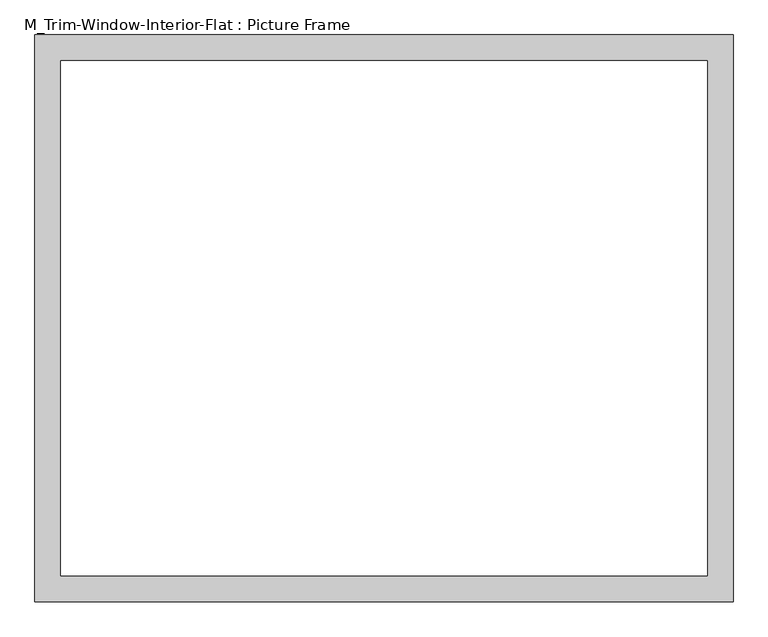
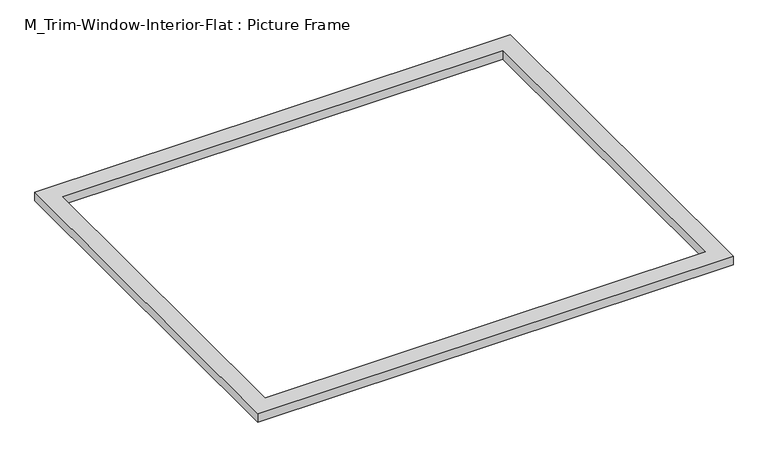
"""IFC4 building model written with IfcOpenShell, lengths in millimetres: proxy geometry, M_Trim-Window-Interior-Flat : Picture Frame."""

import ifcopenshell
import ifcopenshell.guid

model = None  # the IFC model being written
_history = None  # IfcOwnerHistory: only IFC2X3 demands one
_inside = {}  # id of a spatial element -> (the spatial element, [elements in it])
_under = {}  # id of a project, library or spatial element -> (it, [spatial elements below it])
_declared = {}  # id of a project -> (the project, [libraries it declares])
_typed = {}  # id of a type object -> (the type object, [elements of that type])
_made_of = {}  # id of a material, layer set ... -> (it, [elements and type objects made of it])


def new_model(schema):
    """Start an empty IFC model of exactly this schema.

    Asked for "IFC4X3", IfcOpenShell would pick the latest addendum, in which some entities
    have other attributes; the version numbers below select the first issue.
    IFC2X3 requires an IfcOwnerHistory on every rooted entity: one is made here for all.
    """
    global model, _history
    if schema == "IFC4X3":
        model = ifcopenshell.file(schema_version=(4, 3, 0, 0))
    else:
        model = ifcopenshell.file(schema=schema)
    _inside.clear()
    _under.clear()
    _declared.clear()
    _typed.clear()
    _made_of.clear()
    _history = None
    if model.schema == "IFC2X3":
        org = make("IfcOrganization", Name="unknown")
        user = make(
            "IfcPersonAndOrganization",
            ThePerson=make("IfcPerson", FamilyName="unknown"),
            TheOrganization=org,
        )
        app = make(
            "IfcApplication",
            ApplicationDeveloper=org,
            Version="unknown",
            ApplicationFullName="unknown",
            ApplicationIdentifier="unknown",
        )
        _history = make(
            "IfcOwnerHistory",
            OwningUser=user,
            OwningApplication=app,
            ChangeAction="ADDED",
            CreationDate=0,
        )
    return model


def make(cls, **values):
    """One entity of the class cls with the attributes given. An attribute that is None is left unset."""
    return model.create_entity(
        cls, **{name: value for name, value in values.items() if value is not None}
    )


def rooted(cls, **values):
    """An entity with a GlobalId (a new one), such as an element, a storey or a relation."""
    return make(cls, GlobalId=ifcopenshell.guid.new(), OwnerHistory=_history, **values)


def si_unit(unit_type, name, prefix=None):
    """IfcSIUnit, for example si_unit("LENGTHUNIT", "METRE", prefix="MILLI")."""
    return make("IfcSIUnit", UnitType=unit_type, Prefix=prefix, Name=name)


def assignment(units):
    """IfcUnitAssignment: the units of a project."""
    return None if units is None else make("IfcUnitAssignment", Units=units)


def point(xyz):
    """IfcCartesianPoint."""
    return None if xyz is None else make("IfcCartesianPoint", Coordinates=xyz)


def direction(xyz):
    """IfcDirection."""
    return None if xyz is None else make("IfcDirection", DirectionRatios=xyz)


def frame(location, z_axis=None, x_axis=None):
    """IfcAxis2Placement3D, a coordinate frame: its origin and axes. An axis left out is left unset."""
    return make(
        "IfcAxis2Placement3D",
        Location=point(location),
        Axis=direction(z_axis),
        RefDirection=direction(x_axis),
    )


def origin():
    """The frame at (0, 0, 0) with its axes left unset."""
    return frame((0.0, 0.0, 0.0))


def origin_with_axes():
    """The frame at (0, 0, 0) with the z axis (0, 0, 1) and the x axis (1, 0, 0) written out."""
    return frame((0.0, 0.0, 0.0), z_axis=(0.0, 0.0, 1.0), x_axis=(1.0, 0.0, 0.0))


def place(relative_to, where):
    """IfcLocalPlacement: puts the frame where relative to a parent placement (None: the world)."""
    return make(
        "IfcLocalPlacement", PlacementRelTo=relative_to, RelativePlacement=where
    )


def context(
    kind, dimensions, precision=None, world=None, true_north=None, identifier=None
):
    """IfcGeometricRepresentationContext, for example the 3D "Model" context."""
    return make(
        "IfcGeometricRepresentationContext",
        ContextIdentifier=identifier,
        ContextType=kind,
        CoordinateSpaceDimension=dimensions,
        Precision=precision,
        WorldCoordinateSystem=world,
        TrueNorth=true_north,
    )


def project(units=None, contexts=None):
    """IfcProject with its units and contexts."""
    return rooted(
        "IfcProject",
        Name="project",
        RepresentationContexts=contexts,
        UnitsInContext=assignment(units),
    )


def spatial(cls, under=None, at=None, **own):
    """A site, building, storey or space (cls), placed at a placement, below another one or the project."""
    s = rooted(cls, ObjectPlacement=at, **own)
    if under is not None:
        _under.setdefault(under.id(), (under, []))[1].append(s)
    return s


def polyline(points):
    """IfcPolyline through the points."""
    return make("IfcPolyline", Points=[point(p) for p in points])


def outline(outer, holes=None, kind="AREA"):
    """IfcArbitraryClosedProfileDef: a profile drawn as a closed curve; with holes, ...WithVoids."""
    if holes is None:
        return make("IfcArbitraryClosedProfileDef", ProfileType=kind, OuterCurve=outer)
    return make(
        "IfcArbitraryProfileDefWithVoids",
        ProfileType=kind,
        OuterCurve=outer,
        InnerCurves=holes,
    )


def extrude(swept, where, along, depth):
    """IfcExtrudedAreaSolid: the profile swept, set in the frame where, extruded along a direction by depth."""
    return make(
        "IfcExtrudedAreaSolid",
        SweptArea=swept,
        Position=where,
        ExtrudedDirection=direction(along),
        Depth=depth,
    )


def shape(context_of_items, identifier, shape_type, items):
    """IfcShapeRepresentation: the items that make up one representation, for example the "Body"."""
    return make(
        "IfcShapeRepresentation",
        ContextOfItems=context_of_items,
        RepresentationIdentifier=identifier,
        RepresentationType=shape_type,
        Items=items,
    )


def source(mapping_origin, context_of_items, identifier, shape_type, items):
    """IfcRepresentationMap: a shape defined once, which mapped items show again and again."""
    return make(
        "IfcRepresentationMap",
        MappingOrigin=mapping_origin,
        MappedRepresentation=shape(context_of_items, identifier, shape_type, items),
    )


def transform(
    local_origin,
    x_axis=None,
    y_axis=None,
    z_axis=None,
    scale=None,
    scale2=None,
    scale3=None,
    uniform=True,
):
    """IfcCartesianTransformationOperator3D, or its non-uniform kind. x_axis, y_axis, z_axis: its Axis1, 2, 3."""
    if uniform:
        return make(
            "IfcCartesianTransformationOperator3D",
            Axis1=direction(x_axis),
            Axis2=direction(y_axis),
            LocalOrigin=point(local_origin),
            Scale=scale,
            Axis3=direction(z_axis),
        )
    return make(
        "IfcCartesianTransformationOperator3DnonUniform",
        Axis1=direction(x_axis),
        Axis2=direction(y_axis),
        LocalOrigin=point(local_origin),
        Scale=scale,
        Axis3=direction(z_axis),
        Scale2=scale2,
        Scale3=scale3,
    )


def mapped(mapping_source, mapping_target):
    """IfcMappedItem: shows the shape of a source again, moved by a transform."""
    return make(
        "IfcMappedItem", MappingSource=mapping_source, MappingTarget=mapping_target
    )


def made_of(thing, what):
    """Note that an element or type object is made of a material, layer set ...; save() writes the relation."""
    if what is not None:
        _made_of.setdefault(what.id(), (what, []))[1].append(thing)
    return thing


def element(
    cls,
    number,
    at=None,
    inside=None,
    cuts=None,
    type_object=None,
    material=None,
    context=None,
    identifier="Body",
    shape_type=None,
    held_by="IfcProductDefinitionShape",
    body=None,
    shapes=None,
    **own,
):
    """One element of the class cls, such as IfcWall. Its Tag is "e" and its number.

    at: its placement. inside: the storey or other place that contains it. cuts: it is an
    opening in that element (IfcRelVoidsElement). A single representation is given by context,
    identifier, shape_type and body (its items); several are given by shapes. held_by: the class
    of the entity that holds the representations. save() writes the other relations.
    """
    e = rooted(cls, Tag="e%d" % number, ObjectPlacement=at, **own)
    if body is not None:
        shapes = [shape(context, identifier, shape_type, body)]
    if shapes is not None:
        e.Representation = make(held_by, Representations=shapes)
    if inside is not None:
        _inside.setdefault(inside.id(), (inside, []))[1].append(e)
    if cuts is not None:
        rooted(
            "IfcRelVoidsElement", RelatingBuildingElement=cuts, RelatedOpeningElement=e
        )
    if type_object is not None:
        _typed.setdefault(type_object.id(), (type_object, []))[1].append(e)
    return made_of(e, material)


def aggregate(whole, parts):
    """IfcRelAggregates: a whole, such as a stair, and the parts it consists of."""
    return rooted("IfcRelAggregates", RelatingObject=whole, RelatedObjects=parts)


def save(model, path):
    """Write the relations noted so far, then the file.

    IfcRelAggregates (storeys below a building ...), IfcRelContainedInSpatialStructure (elements
    in a storey), IfcRelDefinesByType, IfcRelAssociatesMaterial and IfcRelDeclares: one each for
    every whole, place, type object, material and project.
    """
    for whole, parts in _under.values():
        aggregate(whole, parts)
    for where, things in _inside.values():
        rooted(
            "IfcRelContainedInSpatialStructure",
            RelatedElements=things,
            RelatingStructure=where,
        )
    for kind, things in _typed.values():
        rooted("IfcRelDefinesByType", RelatedObjects=things, RelatingType=kind)
    for what, things in _made_of.values():
        rooted("IfcRelAssociatesMaterial", RelatedObjects=things, RelatingMaterial=what)
    for by, libraries in _declared.values():
        rooted("IfcRelDeclares", RelatingContext=by, RelatedDefinitions=libraries)
    model.write(path)


def m_trim_window_interior_flat_picture_frame_47b855ed(model_context):
    return source(origin(), model_context, "Body", "SweptSolid", [
        extrude(outline(polyline([(809.3, 47.3), (809.3, -1266.5), (-809.3, -1266.5), (-809.3, 47.3), (809.3, 47.3)]), holes=[polyline([(749.3, -12.7), (-749.3, -12.7), (-749.3, -1206.5), (749.3, -1206.5), (749.3, -12.7)])]), origin_with_axes(), (0.0, 0.0, 1.0), 30.0),
    ])


if __name__ == "__main__":
    model = new_model("IFC4")
    model_context = context("Model", 3, world=origin())
    ifc_project = project(units=[si_unit("LENGTHUNIT", "METRE", prefix="MILLI")], contexts=[model_context])
    site = spatial("IfcSite", under=ifc_project)
    building = spatial("IfcBuilding", under=site)
    placement = place(None, origin())
    m_trim_window_interior_flat_picture_frame_shape = m_trim_window_interior_flat_picture_frame_47b855ed(model_context)
    element("IfcBuildingElementProxy", 1, Name="M_Trim-Window-Interior-Flat : Picture Frame", ObjectType="M_Trim-Window-Interior-Flat : Picture Frame", at=placement, inside=building, context=model_context, shape_type="MappedRepresentation", body=[
        mapped(m_trim_window_interior_flat_picture_frame_shape, transform((0.0, 0.0, 0.0), x_axis=(1.0, 0.0, 0.0), y_axis=(0.0, 1.0, 0.0), z_axis=(0.0, 0.0, 1.0))),
    ])
    save(model, "model.ifc")

# Revit data of these elements
# Type "M_Trim-Window-Interior-Flat : Picture Frame"
#   Trim Thickness_Picture Frame = 0' - 1.1811"
#   Trim Width = 0' - 2.3622"
#   Trim Thickness_with Sill = 0' - 0.7874"
#   Sill Thickness = 0' - 1.1811"
#   Opening Width [instance default] = 1' - 11.62205"
#   Opening Height [instance default] = 2' - 11.43307"
#   Default Elevation = 3' - 11.24409"
#   Sill = no
#   Picture Frame = yes
#   Trim Material [instance default] = none
# Element 1 (IfcBuildingElementProxy, "M_Trim-Window-Interior-Flat : Picture Frame")
#   Opening Width = 5' - 0"
#   Opening Height = 4' - 0"
#   Trim Material = Wood - Stained
#   Materials on its faces: "Wood - Stained"
# Materials
#   "Wood - Stained": class "Wood", colour RGB 224 178 126, transparency 0, Cost = 0
